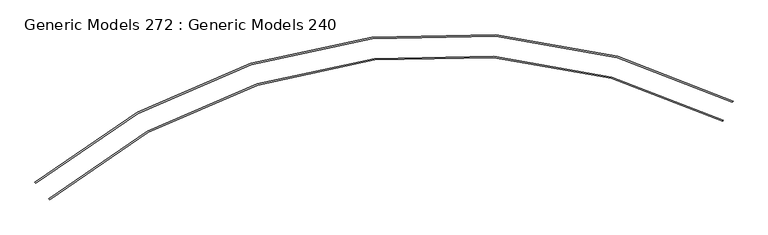
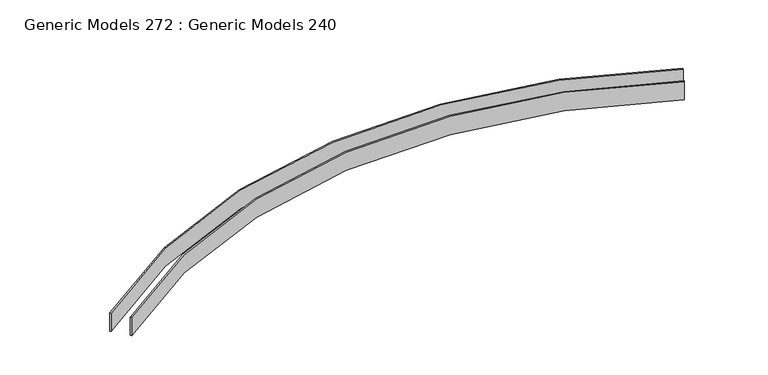
"""IFC4 building model written with IfcOpenShell, lengths in millimetres: proxy geometry, Generic Models 272 : Generic Models 240."""

from ifc_helpers import new_model, si_unit, point, frame_2d, origin, origin_with_axes, place, context, project, spatial, polyline, circle_curve, trimmed, segment, composite_curve, outline, extrude, source, transform, mapped, element, save


def generic_models_272_generic_models_240_170e7ca9(model_context):
    return source(origin(), model_context, "Body", "SweptSolid", [
        extrude(outline(composite_curve([segment(trimmed(circle_curve(frame_2d((-832.04683, -25139.2753781)), 2940.6618053), [point((-2719.4758985, -22884.2580024))], [point((487.9927319, -22511.5411053))], False, "CARTESIAN"), True, "CONTINUOUS"), segment(polyline([(487.9927319, -22511.5411053), (485.1422677, -22517.2153765)]), True, "CONTINUOUS"), segment(trimmed(circle_curve(frame_2d((-832.04683, -25139.2753781)), 2934.3118053), [point((485.1422677, -22517.2153765))], [point((-2715.400226, -22889.127437))], True, "CARTESIAN"), True, "CONTINUOUS"), segment(polyline([(-2715.400226, -22889.127437), (-2719.4758985, -22884.2580024)]), True, "CONTINUOUS")], self_intersect=False)), origin_with_axes(), (0.0, 0.0, 1.0), 101.6),
        extrude(outline(composite_curve([segment(trimmed(circle_curve(frame_2d((-832.04683, -25139.2753781)), 2842.1947981), [point((-2656.2760122, -22959.7664515))], [point((443.79168, -22599.5298461))], False, "CARTESIAN"), True, "CONTINUOUS"), segment(polyline([(443.79168, -22599.5298461), (440.9412158, -22605.2041173)]), True, "CONTINUOUS"), segment(trimmed(circle_curve(frame_2d((-832.04683, -25139.2753781)), 2835.8447981), [point((440.9412158, -22605.2041173))], [point((-2652.2003397, -22964.6358861))], True, "CARTESIAN"), True, "CONTINUOUS"), segment(polyline([(-2652.2003397, -22964.6358861), (-2656.2760122, -22959.7664515)]), True, "CONTINUOUS")], self_intersect=False)), origin_with_axes(), (0.0, 0.0, 1.0), 101.6),
    ])


if __name__ == "__main__":
    model = new_model("IFC4")
    model_context = context("Model", 3, world=origin())
    ifc_project = project(units=[si_unit("LENGTHUNIT", "METRE", prefix="MILLI")], contexts=[model_context])
    site = spatial("IfcSite", under=ifc_project)
    building = spatial("IfcBuilding", under=site)
    placement = place(None, origin())
    generic_models_272_generic_models_240_shape = generic_models_272_generic_models_240_170e7ca9(model_context)
    element("IfcBuildingElementProxy", 1, Name="Generic Models 272 : Generic Models 240", ObjectType="Generic Models 272 : Generic Models 240", at=placement, inside=building, context=model_context, shape_type="MappedRepresentation", body=[
        mapped(generic_models_272_generic_models_240_shape, transform((0.0, 0.0, 0.0), x_axis=(1.0, 0.0, 0.0), y_axis=(0.0, 1.0, 0.0), z_axis=(0.0, 0.0, 1.0))),
    ])
    save(model, "model.ifc")

# Revit data of these elements
# Element 1 (IfcBuildingElementProxy, "Generic Models 272 : Generic Models 240")
#   Materials on its faces: "1/4\" THICK GALVANIZED SHEET METAL"
# Materials
#   "1/4\" THICK GALVANIZED SHEET METAL": class "Unassigned", colour RGB 219 210 213, transparency 0, Keynote = "M05121300.02", Cost = 0
